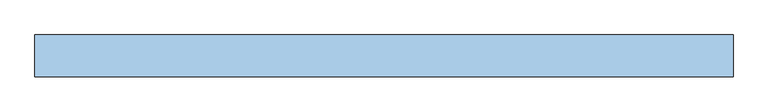
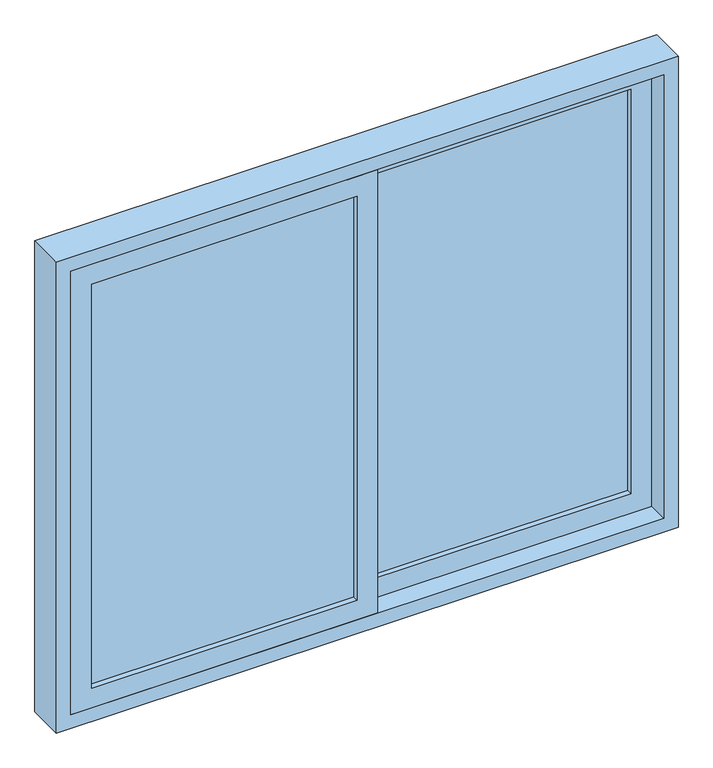
"""IFC4 building model written with IfcOpenShell, lengths in millimetres: window geometry, Janela de correr - 2 Painéis : Janela de correr - 2 Painéis 1,50m."""

import ifcopenshell
import ifcopenshell.guid

model = None  # the IFC model being written
_history = None  # IfcOwnerHistory: only IFC2X3 demands one
_inside = {}  # id of a spatial element -> (the spatial element, [elements in it])
_under = {}  # id of a project, library or spatial element -> (it, [spatial elements below it])
_declared = {}  # id of a project -> (the project, [libraries it declares])
_typed = {}  # id of a type object -> (the type object, [elements of that type])
_made_of = {}  # id of a material, layer set ... -> (it, [elements and type objects made of it])


def new_model(schema):
    """Start an empty IFC model of exactly this schema.

    Asked for "IFC4X3", IfcOpenShell would pick the latest addendum, in which some entities
    have other attributes; the version numbers below select the first issue.
    IFC2X3 requires an IfcOwnerHistory on every rooted entity: one is made here for all.
    """
    global model, _history
    if schema == "IFC4X3":
        model = ifcopenshell.file(schema_version=(4, 3, 0, 0))
    else:
        model = ifcopenshell.file(schema=schema)
    _inside.clear()
    _under.clear()
    _declared.clear()
    _typed.clear()
    _made_of.clear()
    _history = None
    if model.schema == "IFC2X3":
        org = make("IfcOrganization", Name="unknown")
        user = make(
            "IfcPersonAndOrganization",
            ThePerson=make("IfcPerson", FamilyName="unknown"),
            TheOrganization=org,
        )
        app = make(
            "IfcApplication",
            ApplicationDeveloper=org,
            Version="unknown",
            ApplicationFullName="unknown",
            ApplicationIdentifier="unknown",
        )
        _history = make(
            "IfcOwnerHistory",
            OwningUser=user,
            OwningApplication=app,
            ChangeAction="ADDED",
            CreationDate=0,
        )
    return model


def make(cls, **values):
    """One entity of the class cls with the attributes given. An attribute that is None is left unset."""
    return model.create_entity(
        cls, **{name: value for name, value in values.items() if value is not None}
    )


def rooted(cls, **values):
    """An entity with a GlobalId (a new one), such as an element, a storey or a relation."""
    return make(cls, GlobalId=ifcopenshell.guid.new(), OwnerHistory=_history, **values)


def si_unit(unit_type, name, prefix=None):
    """IfcSIUnit, for example si_unit("LENGTHUNIT", "METRE", prefix="MILLI")."""
    return make("IfcSIUnit", UnitType=unit_type, Prefix=prefix, Name=name)


def assignment(units):
    """IfcUnitAssignment: the units of a project."""
    return None if units is None else make("IfcUnitAssignment", Units=units)


def point(xyz):
    """IfcCartesianPoint."""
    return None if xyz is None else make("IfcCartesianPoint", Coordinates=xyz)


def direction(xyz):
    """IfcDirection."""
    return None if xyz is None else make("IfcDirection", DirectionRatios=xyz)


def frame(location, z_axis=None, x_axis=None):
    """IfcAxis2Placement3D, a coordinate frame: its origin and axes. An axis left out is left unset."""
    return make(
        "IfcAxis2Placement3D",
        Location=point(location),
        Axis=direction(z_axis),
        RefDirection=direction(x_axis),
    )


def origin():
    """The frame at (0, 0, 0) with its axes left unset."""
    return frame((0.0, 0.0, 0.0))


def place(relative_to, where):
    """IfcLocalPlacement: puts the frame where relative to a parent placement (None: the world)."""
    return make(
        "IfcLocalPlacement", PlacementRelTo=relative_to, RelativePlacement=where
    )


def context(
    kind, dimensions, precision=None, world=None, true_north=None, identifier=None
):
    """IfcGeometricRepresentationContext, for example the 3D "Model" context."""
    return make(
        "IfcGeometricRepresentationContext",
        ContextIdentifier=identifier,
        ContextType=kind,
        CoordinateSpaceDimension=dimensions,
        Precision=precision,
        WorldCoordinateSystem=world,
        TrueNorth=true_north,
    )


def project(units=None, contexts=None):
    """IfcProject with its units and contexts."""
    return rooted(
        "IfcProject",
        Name="project",
        RepresentationContexts=contexts,
        UnitsInContext=assignment(units),
    )


def spatial(cls, under=None, at=None, **own):
    """A site, building, storey or space (cls), placed at a placement, below another one or the project."""
    s = rooted(cls, ObjectPlacement=at, **own)
    if under is not None:
        _under.setdefault(under.id(), (under, []))[1].append(s)
    return s


def polyline(points):
    """IfcPolyline through the points."""
    return make("IfcPolyline", Points=[point(p) for p in points])


def outline(outer, holes=None, kind="AREA"):
    """IfcArbitraryClosedProfileDef: a profile drawn as a closed curve; with holes, ...WithVoids."""
    if holes is None:
        return make("IfcArbitraryClosedProfileDef", ProfileType=kind, OuterCurve=outer)
    return make(
        "IfcArbitraryProfileDefWithVoids",
        ProfileType=kind,
        OuterCurve=outer,
        InnerCurves=holes,
    )


def extrude(swept, where, along, depth):
    """IfcExtrudedAreaSolid: the profile swept, set in the frame where, extruded along a direction by depth."""
    return make(
        "IfcExtrudedAreaSolid",
        SweptArea=swept,
        Position=where,
        ExtrudedDirection=direction(along),
        Depth=depth,
    )


def shape(context_of_items, identifier, shape_type, items):
    """IfcShapeRepresentation: the items that make up one representation, for example the "Body"."""
    return make(
        "IfcShapeRepresentation",
        ContextOfItems=context_of_items,
        RepresentationIdentifier=identifier,
        RepresentationType=shape_type,
        Items=items,
    )


def source(mapping_origin, context_of_items, identifier, shape_type, items):
    """IfcRepresentationMap: a shape defined once, which mapped items show again and again."""
    return make(
        "IfcRepresentationMap",
        MappingOrigin=mapping_origin,
        MappedRepresentation=shape(context_of_items, identifier, shape_type, items),
    )


def transform(
    local_origin,
    x_axis=None,
    y_axis=None,
    z_axis=None,
    scale=None,
    scale2=None,
    scale3=None,
    uniform=True,
):
    """IfcCartesianTransformationOperator3D, or its non-uniform kind. x_axis, y_axis, z_axis: its Axis1, 2, 3."""
    if uniform:
        return make(
            "IfcCartesianTransformationOperator3D",
            Axis1=direction(x_axis),
            Axis2=direction(y_axis),
            LocalOrigin=point(local_origin),
            Scale=scale,
            Axis3=direction(z_axis),
        )
    return make(
        "IfcCartesianTransformationOperator3DnonUniform",
        Axis1=direction(x_axis),
        Axis2=direction(y_axis),
        LocalOrigin=point(local_origin),
        Scale=scale,
        Axis3=direction(z_axis),
        Scale2=scale2,
        Scale3=scale3,
    )


def mapped(mapping_source, mapping_target):
    """IfcMappedItem: shows the shape of a source again, moved by a transform."""
    return make(
        "IfcMappedItem", MappingSource=mapping_source, MappingTarget=mapping_target
    )


def made_of(thing, what):
    """Note that an element or type object is made of a material, layer set ...; save() writes the relation."""
    if what is not None:
        _made_of.setdefault(what.id(), (what, []))[1].append(thing)
    return thing


def element(
    cls,
    number,
    at=None,
    inside=None,
    cuts=None,
    type_object=None,
    material=None,
    context=None,
    identifier="Body",
    shape_type=None,
    held_by="IfcProductDefinitionShape",
    body=None,
    shapes=None,
    **own,
):
    """One element of the class cls, such as IfcWall. Its Tag is "e" and its number.

    at: its placement. inside: the storey or other place that contains it. cuts: it is an
    opening in that element (IfcRelVoidsElement). A single representation is given by context,
    identifier, shape_type and body (its items); several are given by shapes. held_by: the class
    of the entity that holds the representations. save() writes the other relations.
    """
    e = rooted(cls, Tag="e%d" % number, ObjectPlacement=at, **own)
    if body is not None:
        shapes = [shape(context, identifier, shape_type, body)]
    if shapes is not None:
        e.Representation = make(held_by, Representations=shapes)
    if inside is not None:
        _inside.setdefault(inside.id(), (inside, []))[1].append(e)
    if cuts is not None:
        rooted(
            "IfcRelVoidsElement", RelatingBuildingElement=cuts, RelatedOpeningElement=e
        )
    if type_object is not None:
        _typed.setdefault(type_object.id(), (type_object, []))[1].append(e)
    return made_of(e, material)


def aggregate(whole, parts):
    """IfcRelAggregates: a whole, such as a stair, and the parts it consists of."""
    return rooted("IfcRelAggregates", RelatingObject=whole, RelatedObjects=parts)


def save(model, path):
    """Write the relations noted so far, then the file.

    IfcRelAggregates (storeys below a building ...), IfcRelContainedInSpatialStructure (elements
    in a storey), IfcRelDefinesByType, IfcRelAssociatesMaterial and IfcRelDeclares: one each for
    every whole, place, type object, material and project.
    """
    for whole, parts in _under.values():
        aggregate(whole, parts)
    for where, things in _inside.values():
        rooted(
            "IfcRelContainedInSpatialStructure",
            RelatedElements=things,
            RelatingStructure=where,
        )
    for kind, things in _typed.values():
        rooted("IfcRelDefinesByType", RelatedObjects=things, RelatingType=kind)
    for what, things in _made_of.values():
        rooted("IfcRelAssociatesMaterial", RelatedObjects=things, RelatingMaterial=what)
    for by, libraries in _declared.values():
        rooted("IfcRelDeclares", RelatingContext=by, RelatedDefinitions=libraries)
    model.write(path)


def window_b30dc206(model_context):
    return source(origin(), model_context, "Body", "SweptSolid", [
        extrude(outline(polyline([(685.0, -25.0), (685.0, 715.0), (1815.0, 715.0), (1815.0, -25.0), (685.0, -25.0)]), holes=[polyline([(1765.0, 25.0), (1765.0, 665.0), (735.0, 665.0), (735.0, 25.0), (1765.0, 25.0)])]), frame((0.0, -20.0, 0.0), z_axis=(0.0, 1.0, 0.0), x_axis=(0.0, 0.0, 1.0)), (0.0, 0.0, 1.0), 40.0),
        extrude(outline(polyline([(1815.0, 25.0), (1815.0, -715.0), (685.0, -715.0), (685.0, 25.0), (1815.0, 25.0)]), holes=[polyline([(735.0, -25.0), (735.0, -665.0), (1765.0, -665.0), (1765.0, -25.0), (735.0, -25.0)])]), frame((0.0, -70.0, 0.0), z_axis=(0.0, 1.0, 0.0), x_axis=(0.0, 0.0, 1.0)), (0.0, 0.0, 1.0), 40.0),
        extrude(outline(polyline([(1850.0, 750.0), (1850.0, -750.0), (650.0, -750.0), (650.0, 750.0), (1850.0, 750.0)]), holes=[polyline([(685.0, 715.0), (685.0, -715.0), (1815.0, -715.0), (1815.0, 715.0), (685.0, 715.0)])]), frame((0.0, -70.0, 0.0), z_axis=(0.0, 1.0, 0.0), x_axis=(0.0, 0.0, 1.0)), (0.0, 0.0, 1.0), 90.0),
        extrude(outline(polyline([(25.0, 7.0), (665.0, 7.0), (665.0, -7.0), (25.0, -7.0), (25.0, 7.0)])), frame((0.0, 0.0, 735.0), z_axis=(0.0, 0.0, 1.0), x_axis=(1.0, 0.0, 0.0)), (0.0, 0.0, 1.0), 1030.0),
        extrude(outline(polyline([(-665.0, -43.0), (-25.0, -43.0), (-25.0, -57.0), (-665.0, -57.0), (-665.0, -43.0)])), frame((0.0, 0.0, 735.0), z_axis=(0.0, 0.0, 1.0), x_axis=(1.0, 0.0, 0.0)), (0.0, 0.0, 1.0), 1030.0),
    ])


if __name__ == "__main__":
    model = new_model("IFC4")
    model_context = context("Model", 3, world=origin())
    ifc_project = project(units=[si_unit("LENGTHUNIT", "METRE", prefix="MILLI")], contexts=[model_context])
    site = spatial("IfcSite", under=ifc_project)
    building = spatial("IfcBuilding", under=site)
    placement = place(None, origin())
    window_shape = window_b30dc206(model_context)
    element("IfcWindow", 1, ObjectType="Janela de correr - 2 Painéis : Janela de correr - 2 Painéis 1,50m", at=placement, inside=building, context=model_context, shape_type="MappedRepresentation", body=[
        mapped(window_shape, transform((0.0, 0.0, 0.0), x_axis=(1.0, 0.0, 0.0), y_axis=(0.0, 1.0, 0.0), z_axis=(0.0, 0.0, 1.0))),
    ])
    save(model, "model.ifc")

# Revit data of these elements
# Type "Janela de correr - 2 Painéis : Janela de correr - 2 Painéis 1,50m"
#   Type Mark = "EF29"
#   Construction Type Id = "GSP4R"
#   Analytic Construction = "Vidraça única Pilkington 1/8 pol"
#   Visual Light Transmittance = 0.9
#   Solar Heat Gain Coefficient = 0.78
#   Rough Width = 1.500 m
#   Rough Height = 1.200 m
#   Largura da moldura do painel = 0.050 m
#   Espessura da moldura do painel = 0.040 m
#   Height = 1.200 m
#   Heat Transfer Coefficient (U) = 3.6886 W/(m²·K)
#   Largura da estrutura = 0.035 m
#   Espessura da moldura = 0.090 m
#   Altura-padrão do peitoril = 0.650 m
#   Width = 1.500 m
#   Define Thermal Properties by = 1
#   Vidro = none
#   Material da moldura = none
#   Wall Closure = (empty or 0)
# Element 1 (IfcWindow, "Janela de correr - 2 Painéis : Janela de correr - 2 Painéis 1,50m")
#   Materials on its faces: "Glass"
# Materials
#   "Glass": class "Glass", colour RGB 0 128 192, transparency 0.75, Description = "Soda Lime Glass", Cost = 0
